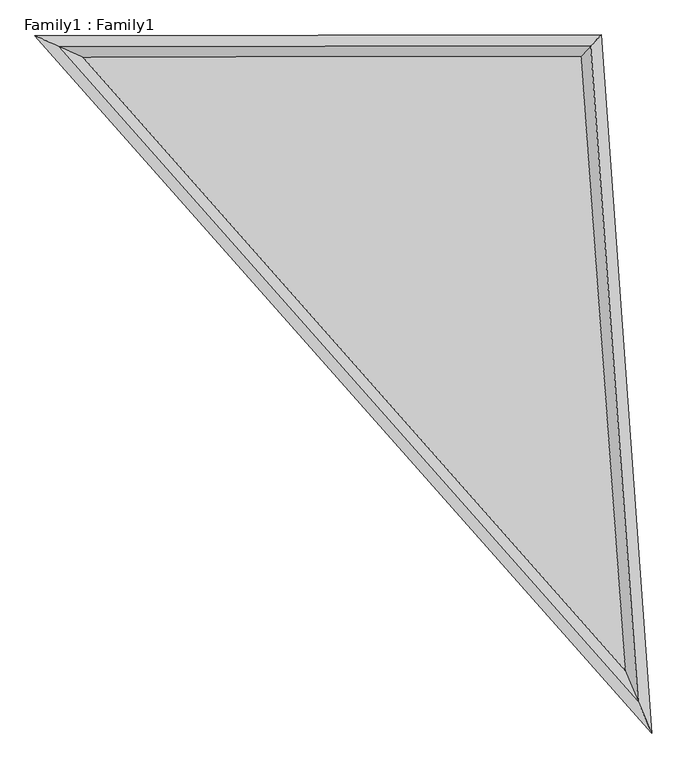
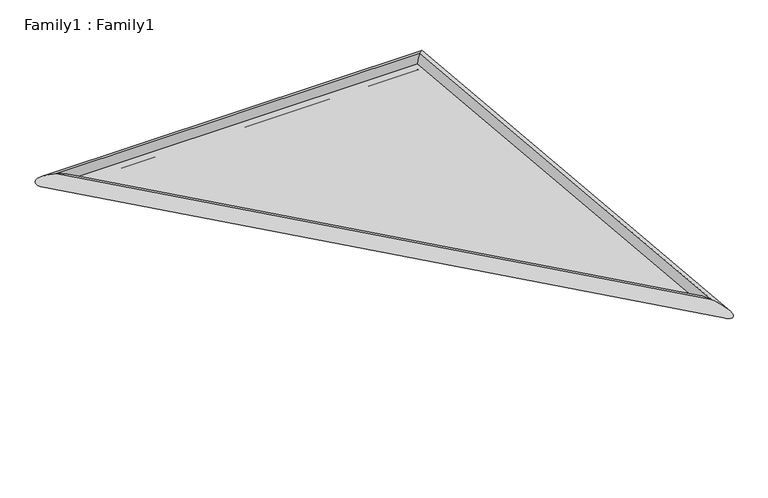
"""IFC4 building model written with IfcOpenShell, lengths in millimetres: proxy geometry, Family1 : Family1."""

from ifc_helpers import new_model, si_unit, frame, origin, origin_with_axes, place, context, project, spatial, polyline, ellipse_curve, outline, extrude, source, transform, mapped, element, save
from ifc_brep_helpers import cylinder_surface, advanced_brep


def family1_family1_c36731b0(model_context):
    return source(origin(), model_context, "Body", "SolidModel", [
        extrude(outline(polyline([(2811.1143728, -3489.6399505), (-2426.699221, 2434.1831391), (2382.5072991, 2439.3980162), (2811.1143728, -3489.6399505)])), origin_with_axes(), (0.0, 0.0, 1.0), 34.1328789),
        advanced_brep(
        [(2811.1143728, -3489.6399505, 100.0), (2811.1143728, -3489.6399505, -100.0), (-2426.699221, 2434.1831391, -100.0), (-2426.699221, 2434.1831391, 100.0), (2382.5072991, 2439.3980162, -100.0), (2382.5072991, 2439.3980162, 100.0)],
        [
            (0, 1, ellipse_curve(frame((2811.1143728, -3489.6399505, 0.0), z_axis=(-0.9218034982538397, -0.38765746556332836, 0.0), x_axis=(0.3876574655633284, -0.9218034982538398, 0.0)), 312.3191938, 100.0)),
            (1, 2),
            (2, 3, ellipse_curve(frame((-2426.699221, 2434.1831391, 0.0), z_axis=(-0.4103601700167169, -0.911923533452148, 0.0), x_axis=(0.9119235334521482, -0.4103601700167171, 0.0)), 243.1027052, 100.0)),
            (3, 0),
            (1, 0, ellipse_curve(frame((2811.1143728, -3489.6399505, 0.0), z_axis=(-0.9218034982538397, -0.38765746556332836, 0.0), x_axis=(0.3876574655633284, -0.9218034982538398, 0.0)), 312.3191938, 100.0)),
            (3, 2, ellipse_curve(frame((-2426.699221, 2434.1831391, 0.0), z_axis=(-0.4103601700167169, -0.911923533452148, 0.0), x_axis=(0.9119235334521482, -0.4103601700167171, 0.0)), 243.1027052, 100.0)),
            (2, 4),
            (4, 5, ellipse_curve(frame((2382.5072991, 2439.3980162, 0.0), z_axis=(-0.7325239999651824, 0.6807412059476122, 0.0), x_axis=(-0.6807412059476122, -0.7325239999651824, 0.0)), 136.6520829, 100.0)),
            (5, 3),
            (5, 4, ellipse_curve(frame((2382.5072991, 2439.3980162, 0.0), z_axis=(-0.7325239999651824, 0.6807412059476122, 0.0), x_axis=(-0.6807412059476122, -0.7325239999651824, 0.0)), 136.6520829, 100.0)),
            (4, 1),
            (0, 5),
        ],
        [
            cylinder_surface(frame((2811.1143728, -3489.6399505, 0.0), z_axis=(0.6623971055005617, -0.7491529047026901, 0.0), x_axis=(-0.7491529047026901, -0.6623971055005617, 0.0)), 100.0),
            cylinder_surface(frame((-2426.699221, 2434.1831391, 0.0), z_axis=(-0.9999994120898983, -0.0010843522757382198, 0.0), x_axis=(-0.0010843522757382198, 0.9999994120898983, 0.0)), 100.0),
            cylinder_surface(frame((2382.5072991, 2439.3980162, 0.0), z_axis=(-0.07210133339414361, 0.9973973118686389, 0.0), x_axis=(0.9973973118686389, 0.07210133339414361, 0.0)), 100.0),
        ],
        [
            (0, [[1, 2, 3, 4]]),
            (0, [[5, -4, 6, -2]]),
            (1, [[-3, 7, 8, 9]]),
            (1, [[-6, -9, 10, -7]]),
            (2, [[-8, 11, -1, 12]]),
            (2, [[-10, -12, -5, -11]]),
        ],
    ),
    ])


if __name__ == "__main__":
    model = new_model("IFC4")
    model_context = context("Model", 3, world=origin())
    ifc_project = project(units=[si_unit("LENGTHUNIT", "METRE", prefix="MILLI")], contexts=[model_context])
    site = spatial("IfcSite", under=ifc_project)
    building = spatial("IfcBuilding", under=site)
    placement = place(None, origin())
    family1_family1_shape = family1_family1_c36731b0(model_context)
    element("IfcBuildingElementProxy", 1, Name="Family1 : Family1", ObjectType="Family1 : Family1", at=placement, inside=building, context=model_context, shape_type="MappedRepresentation", body=[
        mapped(family1_family1_shape, transform((0.0, 0.0, 0.0), x_axis=(1.0, 0.0, 0.0), y_axis=(0.0, 1.0, 0.0), z_axis=(0.0, 0.0, 1.0))),
    ])
    save(model, "model.ifc")

# Revit data of these elements
# Type "Family1 : Family1"
#   Default Elevation = 0
# Element 1 (IfcBuildingElementProxy, "Family1 : Family1")
#   Materials on its faces: "Glass"
# Materials
#   "Glass": class "Glass", colour RGB 0 128 192, transparency 0.9, Description = "Soda Lime Glass", Cost = 0
